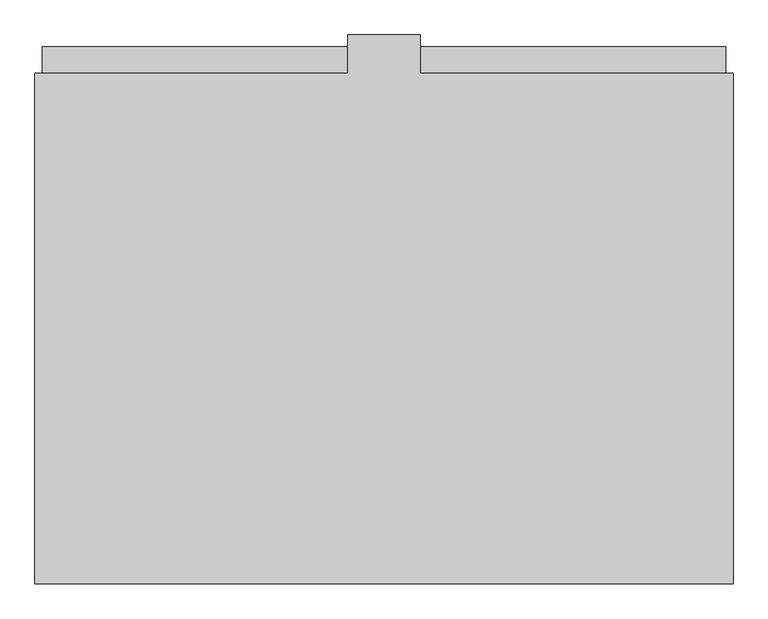
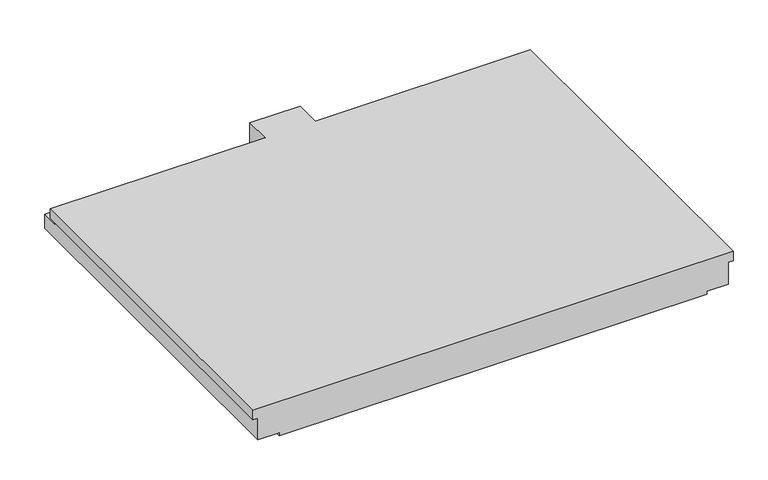
"""IFC4 building model written with IfcOpenShell, lengths in millimetres: stair geometry, NLRS_24_GM_UN_rechthoekig bordes prefab-AV_gen_rsf : prefab bordes_gen__2250x2925."""

import ifcopenshell
import ifcopenshell.guid

model = None  # the IFC model being written
_history = None  # IfcOwnerHistory: only IFC2X3 demands one
_inside = {}  # id of a spatial element -> (the spatial element, [elements in it])
_under = {}  # id of a project, library or spatial element -> (it, [spatial elements below it])
_declared = {}  # id of a project -> (the project, [libraries it declares])
_typed = {}  # id of a type object -> (the type object, [elements of that type])
_made_of = {}  # id of a material, layer set ... -> (it, [elements and type objects made of it])


def new_model(schema):
    """Start an empty IFC model of exactly this schema.

    Asked for "IFC4X3", IfcOpenShell would pick the latest addendum, in which some entities
    have other attributes; the version numbers below select the first issue.
    IFC2X3 requires an IfcOwnerHistory on every rooted entity: one is made here for all.
    """
    global model, _history
    if schema == "IFC4X3":
        model = ifcopenshell.file(schema_version=(4, 3, 0, 0))
    else:
        model = ifcopenshell.file(schema=schema)
    _inside.clear()
    _under.clear()
    _declared.clear()
    _typed.clear()
    _made_of.clear()
    _history = None
    if model.schema == "IFC2X3":
        org = make("IfcOrganization", Name="unknown")
        user = make(
            "IfcPersonAndOrganization",
            ThePerson=make("IfcPerson", FamilyName="unknown"),
            TheOrganization=org,
        )
        app = make(
            "IfcApplication",
            ApplicationDeveloper=org,
            Version="unknown",
            ApplicationFullName="unknown",
            ApplicationIdentifier="unknown",
        )
        _history = make(
            "IfcOwnerHistory",
            OwningUser=user,
            OwningApplication=app,
            ChangeAction="ADDED",
            CreationDate=0,
        )
    return model


def make(cls, **values):
    """One entity of the class cls with the attributes given. An attribute that is None is left unset."""
    return model.create_entity(
        cls, **{name: value for name, value in values.items() if value is not None}
    )


def rooted(cls, **values):
    """An entity with a GlobalId (a new one), such as an element, a storey or a relation."""
    return make(cls, GlobalId=ifcopenshell.guid.new(), OwnerHistory=_history, **values)


def si_unit(unit_type, name, prefix=None):
    """IfcSIUnit, for example si_unit("LENGTHUNIT", "METRE", prefix="MILLI")."""
    return make("IfcSIUnit", UnitType=unit_type, Prefix=prefix, Name=name)


def assignment(units):
    """IfcUnitAssignment: the units of a project."""
    return None if units is None else make("IfcUnitAssignment", Units=units)


def point(xyz):
    """IfcCartesianPoint."""
    return None if xyz is None else make("IfcCartesianPoint", Coordinates=xyz)


def direction(xyz):
    """IfcDirection."""
    return None if xyz is None else make("IfcDirection", DirectionRatios=xyz)


def frame(location, z_axis=None, x_axis=None):
    """IfcAxis2Placement3D, a coordinate frame: its origin and axes. An axis left out is left unset."""
    return make(
        "IfcAxis2Placement3D",
        Location=point(location),
        Axis=direction(z_axis),
        RefDirection=direction(x_axis),
    )


def origin():
    """The frame at (0, 0, 0) with its axes left unset."""
    return frame((0.0, 0.0, 0.0))


def place(relative_to, where):
    """IfcLocalPlacement: puts the frame where relative to a parent placement (None: the world)."""
    return make(
        "IfcLocalPlacement", PlacementRelTo=relative_to, RelativePlacement=where
    )


def context(
    kind, dimensions, precision=None, world=None, true_north=None, identifier=None
):
    """IfcGeometricRepresentationContext, for example the 3D "Model" context."""
    return make(
        "IfcGeometricRepresentationContext",
        ContextIdentifier=identifier,
        ContextType=kind,
        CoordinateSpaceDimension=dimensions,
        Precision=precision,
        WorldCoordinateSystem=world,
        TrueNorth=true_north,
    )


def project(units=None, contexts=None):
    """IfcProject with its units and contexts."""
    return rooted(
        "IfcProject",
        Name="project",
        RepresentationContexts=contexts,
        UnitsInContext=assignment(units),
    )


def spatial(cls, under=None, at=None, **own):
    """A site, building, storey or space (cls), placed at a placement, below another one or the project."""
    s = rooted(cls, ObjectPlacement=at, **own)
    if under is not None:
        _under.setdefault(under.id(), (under, []))[1].append(s)
    return s


def faces_of(points, faces, orient=None, outer=None):
    """IfcFace entities. A face is a list of loops; a loop is a list of indices into points, from 0.

    orient and outer hold one flag for each loop. By default every Orientation is true, the
    first loop of a face is its IfcFaceOuterBound and the others are IfcFaceBound.
    """
    made = []
    for i, loops in enumerate(faces):
        bounds = []
        for j, loop in enumerate(loops):
            is_outer = j == 0 if outer is None else outer[i][j]
            bounds.append(
                make(
                    "IfcFaceOuterBound" if is_outer else "IfcFaceBound",
                    Bound=make("IfcPolyLoop", Polygon=[points[k] for k in loop]),
                    Orientation=True if orient is None else orient[i][j],
                )
            )
        made.append(make("IfcFace", Bounds=bounds))
    return made


def faceted_brep(points, faces, orient=None, outer=None, voids=None):
    """IfcFacetedBrep: a solid bounded by flat faces; with voids (closed shells), ...WithVoids."""
    shared = [point(p) for p in points]
    hull = make("IfcClosedShell", CfsFaces=faces_of(shared, faces, orient, outer))
    if voids is None:
        return make("IfcFacetedBrep", Outer=hull)
    return make(
        "IfcFacetedBrepWithVoids",
        Outer=hull,
        Voids=[
            make(cls, CfsFaces=faces_of(shared, fs, o, b)) for cls, fs, o, b in voids
        ],
    )


def shape(context_of_items, identifier, shape_type, items):
    """IfcShapeRepresentation: the items that make up one representation, for example the "Body"."""
    return make(
        "IfcShapeRepresentation",
        ContextOfItems=context_of_items,
        RepresentationIdentifier=identifier,
        RepresentationType=shape_type,
        Items=items,
    )


def source(mapping_origin, context_of_items, identifier, shape_type, items):
    """IfcRepresentationMap: a shape defined once, which mapped items show again and again."""
    return make(
        "IfcRepresentationMap",
        MappingOrigin=mapping_origin,
        MappedRepresentation=shape(context_of_items, identifier, shape_type, items),
    )


def transform(
    local_origin,
    x_axis=None,
    y_axis=None,
    z_axis=None,
    scale=None,
    scale2=None,
    scale3=None,
    uniform=True,
):
    """IfcCartesianTransformationOperator3D, or its non-uniform kind. x_axis, y_axis, z_axis: its Axis1, 2, 3."""
    if uniform:
        return make(
            "IfcCartesianTransformationOperator3D",
            Axis1=direction(x_axis),
            Axis2=direction(y_axis),
            LocalOrigin=point(local_origin),
            Scale=scale,
            Axis3=direction(z_axis),
        )
    return make(
        "IfcCartesianTransformationOperator3DnonUniform",
        Axis1=direction(x_axis),
        Axis2=direction(y_axis),
        LocalOrigin=point(local_origin),
        Scale=scale,
        Axis3=direction(z_axis),
        Scale2=scale2,
        Scale3=scale3,
    )


def mapped(mapping_source, mapping_target):
    """IfcMappedItem: shows the shape of a source again, moved by a transform."""
    return make(
        "IfcMappedItem", MappingSource=mapping_source, MappingTarget=mapping_target
    )


def made_of(thing, what):
    """Note that an element or type object is made of a material, layer set ...; save() writes the relation."""
    if what is not None:
        _made_of.setdefault(what.id(), (what, []))[1].append(thing)
    return thing


def element(
    cls,
    number,
    at=None,
    inside=None,
    cuts=None,
    type_object=None,
    material=None,
    context=None,
    identifier="Body",
    shape_type=None,
    held_by="IfcProductDefinitionShape",
    body=None,
    shapes=None,
    **own,
):
    """One element of the class cls, such as IfcWall. Its Tag is "e" and its number.

    at: its placement. inside: the storey or other place that contains it. cuts: it is an
    opening in that element (IfcRelVoidsElement). A single representation is given by context,
    identifier, shape_type and body (its items); several are given by shapes. held_by: the class
    of the entity that holds the representations. save() writes the other relations.
    """
    e = rooted(cls, Tag="e%d" % number, ObjectPlacement=at, **own)
    if body is not None:
        shapes = [shape(context, identifier, shape_type, body)]
    if shapes is not None:
        e.Representation = make(held_by, Representations=shapes)
    if inside is not None:
        _inside.setdefault(inside.id(), (inside, []))[1].append(e)
    if cuts is not None:
        rooted(
            "IfcRelVoidsElement", RelatingBuildingElement=cuts, RelatedOpeningElement=e
        )
    if type_object is not None:
        _typed.setdefault(type_object.id(), (type_object, []))[1].append(e)
    return made_of(e, material)


def aggregate(whole, parts):
    """IfcRelAggregates: a whole, such as a stair, and the parts it consists of."""
    return rooted("IfcRelAggregates", RelatingObject=whole, RelatedObjects=parts)


def save(model, path):
    """Write the relations noted so far, then the file.

    IfcRelAggregates (storeys below a building ...), IfcRelContainedInSpatialStructure (elements
    in a storey), IfcRelDefinesByType, IfcRelAssociatesMaterial and IfcRelDeclares: one each for
    every whole, place, type object, material and project.
    """
    for whole, parts in _under.values():
        aggregate(whole, parts)
    for where, things in _inside.values():
        rooted(
            "IfcRelContainedInSpatialStructure",
            RelatedElements=things,
            RelatingStructure=where,
        )
    for kind, things in _typed.values():
        rooted("IfcRelDefinesByType", RelatedObjects=things, RelatingType=kind)
    for what, things in _made_of.values():
        rooted("IfcRelAssociatesMaterial", RelatedObjects=things, RelatingMaterial=what)
    for by, libraries in _declared.values():
        rooted("IfcRelDeclares", RelatingContext=by, RelatedDefinitions=libraries)
    model.write(path)


def stair_0f5fce95(model_context):
    return source(origin(), model_context, "Body", "Brep", [
        faceted_brep([(1462.5, 2140.0, 0.0), (1462.5, 0.0, 0.0), (1462.5, 0.0, -60.0), (1462.5, 2140.0, -60.0), (152.5, 2250.0, -110.0), (152.5, 2140.0, -110.0), (1432.5, 2140.0, -110.0), (1432.5, 2250.0, -110.0), (152.5, 2140.0, 0.0), (1432.5, 2140.0, -60.0), (152.5, 2300.0, -220.0), (152.5, 2300.0, 0.0), (152.5, 2250.0, -220.0), (-152.5, 2300.0, 0.0), (-152.5, 2300.0, -220.0), (-152.5, 2250.0, -220.0), (-152.5, 2250.0, -110.0), (-152.5, 2140.0, -110.0), (-152.5, 2140.0, 0.0), (-1462.5, 0.0, 0.0), (-1462.5, 2140.0, 0.0), (-1462.5, 2140.0, -60.0), (-1462.5, 0.0, -60.0), (-1302.5, 2250.0, -220.0), (-1302.5, 2250.0, -200.0), (-1432.5, 2250.0, -200.0), (-1432.5, 2250.0, -110.0), (-1432.5, 2140.0, -110.0), (-1432.5, 2140.0, -60.0), (-1432.5, 0.0, -60.0), (-1432.5, 0.0, -200.0), (-1302.5, 0.0, -200.0), (-1302.5, 0.0, -220.0), (1302.5, 0.0, -220.0), (1302.5, 0.0, -200.0), (1432.5, 0.0, -200.0), (1432.5, 0.0, -60.0), (1302.5, 2250.0, -220.0), (1432.5, 2250.0, -200.0), (1302.5, 2250.0, -200.0)], [[[0, 1, 2, 3]], [[4, 5, 6, 7]], [[8, 0, 3, 9, 6, 5]], [[10, 11, 8, 5, 4, 12]], [[13, 14, 15, 16, 17, 18]], [[19, 20, 21, 22]], [[15, 23, 24, 25, 26, 16]], [[16, 26, 27, 17]], [[20, 18, 17, 27, 28, 21]], [[20, 19, 1, 0, 8, 11, 13, 18]], [[19, 22, 29, 30, 31, 32, 33, 34, 35, 36, 2, 1]], [[23, 15, 14, 10, 12, 37, 33, 32]], [[28, 29, 22, 21]], [[25, 30, 29, 28, 27, 26]], [[30, 25, 24, 31]], [[31, 24, 23, 32]], [[36, 9, 3, 2]], [[9, 36, 35, 38, 7, 6]], [[38, 35, 34, 39]], [[39, 34, 33, 37]], [[12, 4, 7, 38, 39, 37]], [[11, 10, 14, 13]]]),
    ])


if __name__ == "__main__":
    model = new_model("IFC4")
    model_context = context("Model", 3, world=origin())
    ifc_project = project(units=[si_unit("LENGTHUNIT", "METRE", prefix="MILLI")], contexts=[model_context])
    site = spatial("IfcSite", under=ifc_project)
    building = spatial("IfcBuilding", under=site)
    placement = place(None, origin())
    stair_shape = stair_0f5fce95(model_context)
    element("IfcStair", 1, ObjectType="NLRS_24_GM_UN_rechthoekig bordes prefab-AV_gen_rsf : prefab bordes_gen__2250x2925", at=placement, inside=building, context=model_context, shape_type="MappedRepresentation", body=[
        mapped(stair_shape, transform((0.0, 0.0, 0.0), x_axis=(1.0, 0.0, 0.0), y_axis=(0.0, 1.0, 0.0), z_axis=(0.0, 0.0, 1.0))),
    ])
    save(model, "model.ifc")

# Revit data of these elements
# Type "NLRS_24_GM_UN_rechthoekig bordes prefab-AV_gen_rsf : prefab bordes_gen__2250x2925"
#   IfcExportAs = "IfcStair"
#   Type Comments = " "
#   Model = " "
#   Manufacturer = " "
#   Description = "rechthoekig bordes prefab\r\n1930x4395"
#   Assembly Code = "24.15"
#   Width = 2925 mm
#   Thickness = 220 mm
#   Perimeter = 10450 mm
#   NLRS_C_lengte_02 = 1310 mm
#   NLRS_C_lengte_01 = 1310 mm
#   NLRS_C_hoogte_02 = 110 mm
#   NLRS_C_hoogte_01 = 110 mm
#   NLRS_C_diepte_04 = 2250 mm
#   NLRS_C_diepte_03 = 2250 mm
#   NLRS_C_diepte_02 = 110 mm
#   NLRS_C_diepte_01 = 110 mm
#   Length = 2300 mm
#   Default Elevation = 1219.2 mm
#   Area = 6.7275 m²
#   NLRS_C_materiaal = NLRS_f2_beton prefab_gen_rsf
#   Keynote = ""
# Element 1 (IfcStair, "NLRS_24_GM_UN_rechthoekig bordes prefab-AV_gen_rsf : prefab bordes_gen__2250x2925")
#   Materials on its faces: "NLRS_f2_beton prefab_gen_rsf"
# Materials
#   "NLRS_f2_beton prefab_gen_rsf": class "F - Niet gebakken kunststeen", colour RGB 129 133 118, transparency 0, Keynote = "f2", Manufacturer = "Revit Standards Foundation", URL = "www.revitstandards.org", Description = "beton prefab", Cost = 0
